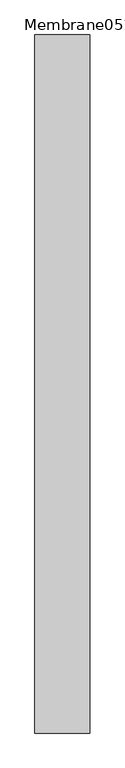
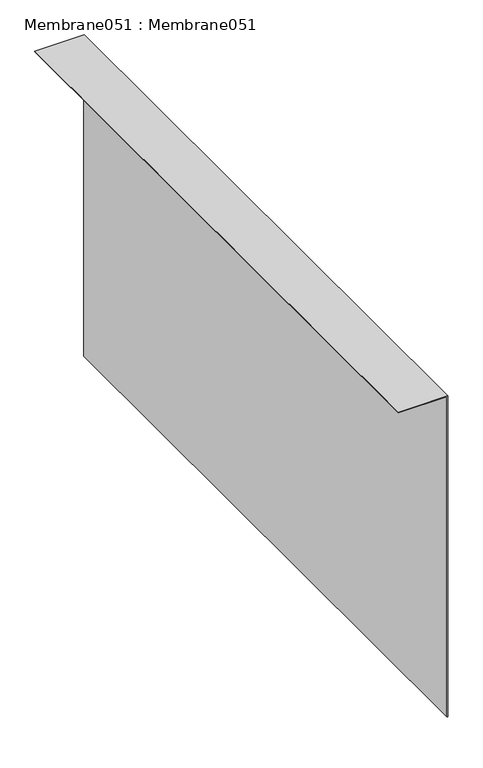
"""IFC4 building model written with IfcOpenShell, lengths in millimetres: proxy geometry, Membrane051 : Membrane051."""

from ifc_helpers import new_model, si_unit, frame, origin, place, context, project, spatial, polyline, outline, extrude, source, transform, mapped, element, save


def membrane051_membrane051_52b596f7(model_context):
    return source(origin(), model_context, "Body", "SweptSolid", [
        extrude(outline(polyline([(33391.6445312, -10088.4443359), (32314.8961275, -10088.4443359), (32314.8961275, -10086.4443359), (33393.6445312, -10086.4443359), (33393.6445312, -10243.8017578), (33391.6445312, -10243.8017578), (33391.6445312, -10088.4443359)])), frame((0.0, 7982.1531721, 0.0), z_axis=(0.0, 1.0, 0.0), x_axis=(0.0, 0.0, 1.0)), (0.0, 0.0, 1.0), 2000.0),
    ])


if __name__ == "__main__":
    model = new_model("IFC4")
    model_context = context("Model", 3, world=origin())
    ifc_project = project(units=[si_unit("LENGTHUNIT", "METRE", prefix="MILLI")], contexts=[model_context])
    site = spatial("IfcSite", under=ifc_project)
    building = spatial("IfcBuilding", under=site)
    placement = place(None, origin())
    membrane051_membrane051_shape = membrane051_membrane051_52b596f7(model_context)
    element("IfcBuildingElementProxy", 1, Name="Membrane051 : Membrane051", ObjectType="Membrane051 : Membrane051", at=placement, inside=building, context=model_context, shape_type="MappedRepresentation", body=[
        mapped(membrane051_membrane051_shape, transform((0.0, 0.0, 0.0), x_axis=(1.0, 0.0, 0.0), y_axis=(0.0, 1.0, 0.0), z_axis=(0.0, 0.0, 1.0))),
    ])
    save(model, "model.ifc")

# Revit data of these elements
# Type "Membrane051 : Membrane051"
#   NameOverride = "Membrane051"
# Element 1 (IfcBuildingElementProxy, "Membrane051 : Membrane051")
#   Materials on its faces: "ECO ROOT BARRIER"
# Materials
#   "ECO ROOT BARRIER": class "Unassigned", colour RGB 135 255 2, transparency 0
